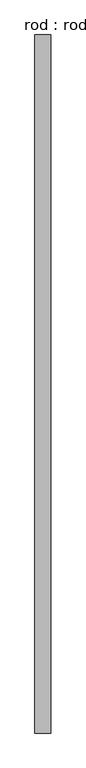
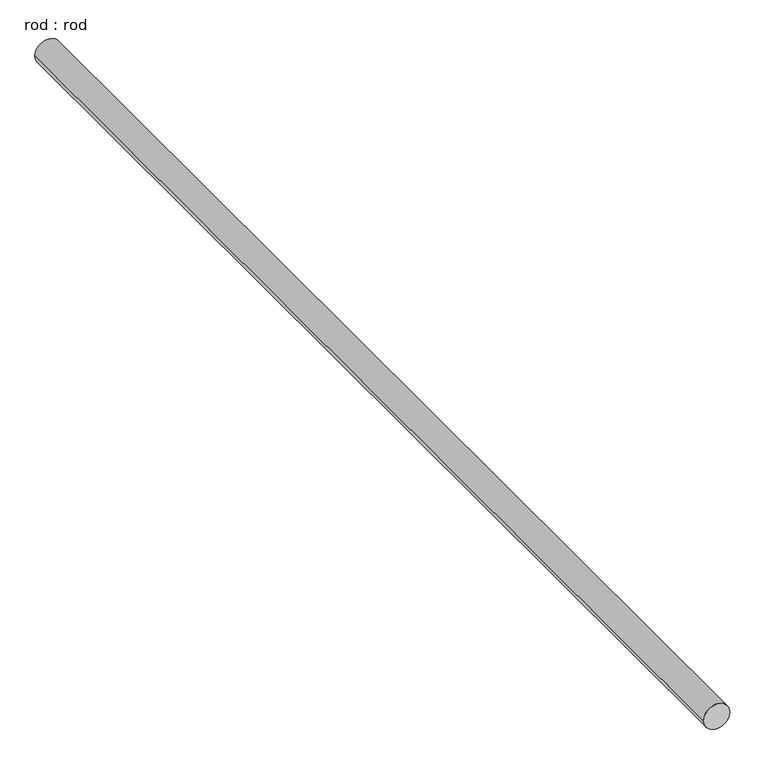
"""IFC4 building model written with IfcOpenShell, lengths in millimetres: proxy geometry, rod : rod."""

from ifc_helpers import new_model, si_unit, point, frame, frame_2d, origin, place, context, project, spatial, circle_curve, trimmed, segment, composite_curve, outline, extrude, source, transform, mapped, element, save


def rod_rod_5be3514e(model_context):
    return source(origin(), model_context, "Body", "SweptSolid", [
        extrude(outline(composite_curve([segment(trimmed(circle_curve(frame_2d((0.0108462, 0.0)), 200.0), [point((0.0108462, 200.0))], [point((0.0108462, -200.0))], False, "CARTESIAN"), True, "CONTINUOUS"), segment(trimmed(circle_curve(frame_2d((0.0108462, 0.0)), 200.0), [point((0.0108462, -200.0))], [point((0.0108462, 200.0))], False, "CARTESIAN"), True, "CONTINUOUS")], self_intersect=False)), frame((0.0, -4748.9558197, 0.0), z_axis=(0.0, 1.0, 0.0), x_axis=(0.0, 0.0, 1.0)), (0.0, 0.0, 1.0), 17683.3688702),
    ])


if __name__ == "__main__":
    model = new_model("IFC4")
    model_context = context("Model", 3, world=origin())
    ifc_project = project(units=[si_unit("LENGTHUNIT", "METRE", prefix="MILLI")], contexts=[model_context])
    site = spatial("IfcSite", under=ifc_project)
    building = spatial("IfcBuilding", under=site)
    placement = place(None, origin())
    rod_rod_shape = rod_rod_5be3514e(model_context)
    element("IfcBuildingElementProxy", 1, Name="rod : rod", ObjectType="rod : rod", at=placement, inside=building, context=model_context, shape_type="MappedRepresentation", body=[
        mapped(rod_rod_shape, transform((0.0, 0.0, 0.0), x_axis=(1.0, 0.0, 0.0), y_axis=(0.0, 1.0, 0.0), z_axis=(0.0, 0.0, 1.0))),
    ])
    save(model, "model.ifc")

# Revit data of these elements
# Type "rod : rod"
#   Default Elevation = 0
